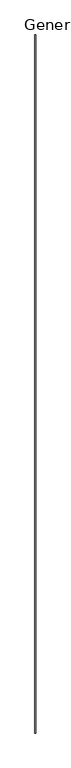
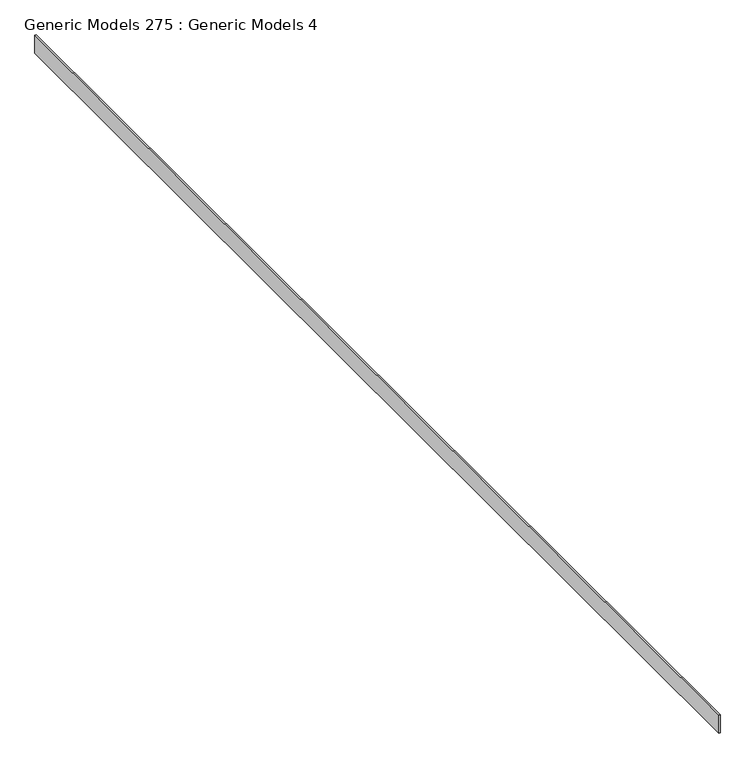
"""IFC4 building model written with IfcOpenShell, lengths in millimetres: proxy geometry, Generic Models 275 : Generic Models 4."""

import ifcopenshell
import ifcopenshell.guid

model = None  # the IFC model being written
_history = None  # IfcOwnerHistory: only IFC2X3 demands one
_inside = {}  # id of a spatial element -> (the spatial element, [elements in it])
_under = {}  # id of a project, library or spatial element -> (it, [spatial elements below it])
_declared = {}  # id of a project -> (the project, [libraries it declares])
_typed = {}  # id of a type object -> (the type object, [elements of that type])
_made_of = {}  # id of a material, layer set ... -> (it, [elements and type objects made of it])


def new_model(schema):
    """Start an empty IFC model of exactly this schema.

    Asked for "IFC4X3", IfcOpenShell would pick the latest addendum, in which some entities
    have other attributes; the version numbers below select the first issue.
    IFC2X3 requires an IfcOwnerHistory on every rooted entity: one is made here for all.
    """
    global model, _history
    if schema == "IFC4X3":
        model = ifcopenshell.file(schema_version=(4, 3, 0, 0))
    else:
        model = ifcopenshell.file(schema=schema)
    _inside.clear()
    _under.clear()
    _declared.clear()
    _typed.clear()
    _made_of.clear()
    _history = None
    if model.schema == "IFC2X3":
        org = make("IfcOrganization", Name="unknown")
        user = make(
            "IfcPersonAndOrganization",
            ThePerson=make("IfcPerson", FamilyName="unknown"),
            TheOrganization=org,
        )
        app = make(
            "IfcApplication",
            ApplicationDeveloper=org,
            Version="unknown",
            ApplicationFullName="unknown",
            ApplicationIdentifier="unknown",
        )
        _history = make(
            "IfcOwnerHistory",
            OwningUser=user,
            OwningApplication=app,
            ChangeAction="ADDED",
            CreationDate=0,
        )
    return model


def make(cls, **values):
    """One entity of the class cls with the attributes given. An attribute that is None is left unset."""
    return model.create_entity(
        cls, **{name: value for name, value in values.items() if value is not None}
    )


def rooted(cls, **values):
    """An entity with a GlobalId (a new one), such as an element, a storey or a relation."""
    return make(cls, GlobalId=ifcopenshell.guid.new(), OwnerHistory=_history, **values)


def si_unit(unit_type, name, prefix=None):
    """IfcSIUnit, for example si_unit("LENGTHUNIT", "METRE", prefix="MILLI")."""
    return make("IfcSIUnit", UnitType=unit_type, Prefix=prefix, Name=name)


def assignment(units):
    """IfcUnitAssignment: the units of a project."""
    return None if units is None else make("IfcUnitAssignment", Units=units)


def point(xyz):
    """IfcCartesianPoint."""
    return None if xyz is None else make("IfcCartesianPoint", Coordinates=xyz)


def direction(xyz):
    """IfcDirection."""
    return None if xyz is None else make("IfcDirection", DirectionRatios=xyz)


def frame(location, z_axis=None, x_axis=None):
    """IfcAxis2Placement3D, a coordinate frame: its origin and axes. An axis left out is left unset."""
    return make(
        "IfcAxis2Placement3D",
        Location=point(location),
        Axis=direction(z_axis),
        RefDirection=direction(x_axis),
    )


def origin():
    """The frame at (0, 0, 0) with its axes left unset."""
    return frame((0.0, 0.0, 0.0))


def place(relative_to, where):
    """IfcLocalPlacement: puts the frame where relative to a parent placement (None: the world)."""
    return make(
        "IfcLocalPlacement", PlacementRelTo=relative_to, RelativePlacement=where
    )


def context(
    kind, dimensions, precision=None, world=None, true_north=None, identifier=None
):
    """IfcGeometricRepresentationContext, for example the 3D "Model" context."""
    return make(
        "IfcGeometricRepresentationContext",
        ContextIdentifier=identifier,
        ContextType=kind,
        CoordinateSpaceDimension=dimensions,
        Precision=precision,
        WorldCoordinateSystem=world,
        TrueNorth=true_north,
    )


def project(units=None, contexts=None):
    """IfcProject with its units and contexts."""
    return rooted(
        "IfcProject",
        Name="project",
        RepresentationContexts=contexts,
        UnitsInContext=assignment(units),
    )


def spatial(cls, under=None, at=None, **own):
    """A site, building, storey or space (cls), placed at a placement, below another one or the project."""
    s = rooted(cls, ObjectPlacement=at, **own)
    if under is not None:
        _under.setdefault(under.id(), (under, []))[1].append(s)
    return s


def polyline(points):
    """IfcPolyline through the points."""
    return make("IfcPolyline", Points=[point(p) for p in points])


def outline(outer, holes=None, kind="AREA"):
    """IfcArbitraryClosedProfileDef: a profile drawn as a closed curve; with holes, ...WithVoids."""
    if holes is None:
        return make("IfcArbitraryClosedProfileDef", ProfileType=kind, OuterCurve=outer)
    return make(
        "IfcArbitraryProfileDefWithVoids",
        ProfileType=kind,
        OuterCurve=outer,
        InnerCurves=holes,
    )


def extrude(swept, where, along, depth):
    """IfcExtrudedAreaSolid: the profile swept, set in the frame where, extruded along a direction by depth."""
    return make(
        "IfcExtrudedAreaSolid",
        SweptArea=swept,
        Position=where,
        ExtrudedDirection=direction(along),
        Depth=depth,
    )


def shape(context_of_items, identifier, shape_type, items):
    """IfcShapeRepresentation: the items that make up one representation, for example the "Body"."""
    return make(
        "IfcShapeRepresentation",
        ContextOfItems=context_of_items,
        RepresentationIdentifier=identifier,
        RepresentationType=shape_type,
        Items=items,
    )


def source(mapping_origin, context_of_items, identifier, shape_type, items):
    """IfcRepresentationMap: a shape defined once, which mapped items show again and again."""
    return make(
        "IfcRepresentationMap",
        MappingOrigin=mapping_origin,
        MappedRepresentation=shape(context_of_items, identifier, shape_type, items),
    )


def transform(
    local_origin,
    x_axis=None,
    y_axis=None,
    z_axis=None,
    scale=None,
    scale2=None,
    scale3=None,
    uniform=True,
):
    """IfcCartesianTransformationOperator3D, or its non-uniform kind. x_axis, y_axis, z_axis: its Axis1, 2, 3."""
    if uniform:
        return make(
            "IfcCartesianTransformationOperator3D",
            Axis1=direction(x_axis),
            Axis2=direction(y_axis),
            LocalOrigin=point(local_origin),
            Scale=scale,
            Axis3=direction(z_axis),
        )
    return make(
        "IfcCartesianTransformationOperator3DnonUniform",
        Axis1=direction(x_axis),
        Axis2=direction(y_axis),
        LocalOrigin=point(local_origin),
        Scale=scale,
        Axis3=direction(z_axis),
        Scale2=scale2,
        Scale3=scale3,
    )


def mapped(mapping_source, mapping_target):
    """IfcMappedItem: shows the shape of a source again, moved by a transform."""
    return make(
        "IfcMappedItem", MappingSource=mapping_source, MappingTarget=mapping_target
    )


def made_of(thing, what):
    """Note that an element or type object is made of a material, layer set ...; save() writes the relation."""
    if what is not None:
        _made_of.setdefault(what.id(), (what, []))[1].append(thing)
    return thing


def element(
    cls,
    number,
    at=None,
    inside=None,
    cuts=None,
    type_object=None,
    material=None,
    context=None,
    identifier="Body",
    shape_type=None,
    held_by="IfcProductDefinitionShape",
    body=None,
    shapes=None,
    **own,
):
    """One element of the class cls, such as IfcWall. Its Tag is "e" and its number.

    at: its placement. inside: the storey or other place that contains it. cuts: it is an
    opening in that element (IfcRelVoidsElement). A single representation is given by context,
    identifier, shape_type and body (its items); several are given by shapes. held_by: the class
    of the entity that holds the representations. save() writes the other relations.
    """
    e = rooted(cls, Tag="e%d" % number, ObjectPlacement=at, **own)
    if body is not None:
        shapes = [shape(context, identifier, shape_type, body)]
    if shapes is not None:
        e.Representation = make(held_by, Representations=shapes)
    if inside is not None:
        _inside.setdefault(inside.id(), (inside, []))[1].append(e)
    if cuts is not None:
        rooted(
            "IfcRelVoidsElement", RelatingBuildingElement=cuts, RelatedOpeningElement=e
        )
    if type_object is not None:
        _typed.setdefault(type_object.id(), (type_object, []))[1].append(e)
    return made_of(e, material)


def aggregate(whole, parts):
    """IfcRelAggregates: a whole, such as a stair, and the parts it consists of."""
    return rooted("IfcRelAggregates", RelatingObject=whole, RelatedObjects=parts)


def save(model, path):
    """Write the relations noted so far, then the file.

    IfcRelAggregates (storeys below a building ...), IfcRelContainedInSpatialStructure (elements
    in a storey), IfcRelDefinesByType, IfcRelAssociatesMaterial and IfcRelDeclares: one each for
    every whole, place, type object, material and project.
    """
    for whole, parts in _under.values():
        aggregate(whole, parts)
    for where, things in _inside.values():
        rooted(
            "IfcRelContainedInSpatialStructure",
            RelatedElements=things,
            RelatingStructure=where,
        )
    for kind, things in _typed.values():
        rooted("IfcRelDefinesByType", RelatedObjects=things, RelatingType=kind)
    for what, things in _made_of.values():
        rooted("IfcRelAssociatesMaterial", RelatedObjects=things, RelatingMaterial=what)
    for by, libraries in _declared.values():
        rooted("IfcRelDeclares", RelatingContext=by, RelatedDefinitions=libraries)
    model.write(path)


def generic_models_275_generic_models_4_c0c91c90(model_context):
    return source(origin(), model_context, "Body", "SweptSolid", [
        extrude(outline(polyline([(1672.1675572, -6864.9230338), (1653.1175572, -6864.9230338), (1653.1175572, 11778.6769662), (1672.1675572, 11778.6769662), (1672.1675572, -6864.9230338)])), frame((0.0, 0.0, 129139.4988454), z_axis=(0.0, 0.0, 1.0), x_axis=(1.0, 0.0, 0.0)), (0.0, 0.0, 1.0), 296.8862249),
    ])


if __name__ == "__main__":
    model = new_model("IFC4")
    model_context = context("Model", 3, world=origin())
    ifc_project = project(units=[si_unit("LENGTHUNIT", "METRE", prefix="MILLI")], contexts=[model_context])
    site = spatial("IfcSite", under=ifc_project)
    building = spatial("IfcBuilding", under=site)
    placement = place(None, origin())
    generic_models_275_generic_models_4_shape = generic_models_275_generic_models_4_c0c91c90(model_context)
    element("IfcBuildingElementProxy", 1, Name="Generic Models 275 : Generic Models 4", ObjectType="Generic Models 275 : Generic Models 4", at=placement, inside=building, context=model_context, shape_type="MappedRepresentation", body=[
        mapped(generic_models_275_generic_models_4_shape, transform((0.0, 0.0, 0.0), x_axis=(1.0, 0.0, 0.0), y_axis=(0.0, 1.0, 0.0), z_axis=(0.0, 0.0, 1.0))),
    ])
    save(model, "model.ifc")

# Revit data of these elements
# Element 1 (IfcBuildingElementProxy, "Generic Models 275 : Generic Models 4")
#   Materials on its faces: "_FIRE RETARDANT WOOD SIDING T.B.D"
# Materials
#   "_FIRE RETARDANT WOOD SIDING T.B.D": class "Generic", colour RGB 177 130 114, transparency 0, Cost = 0
